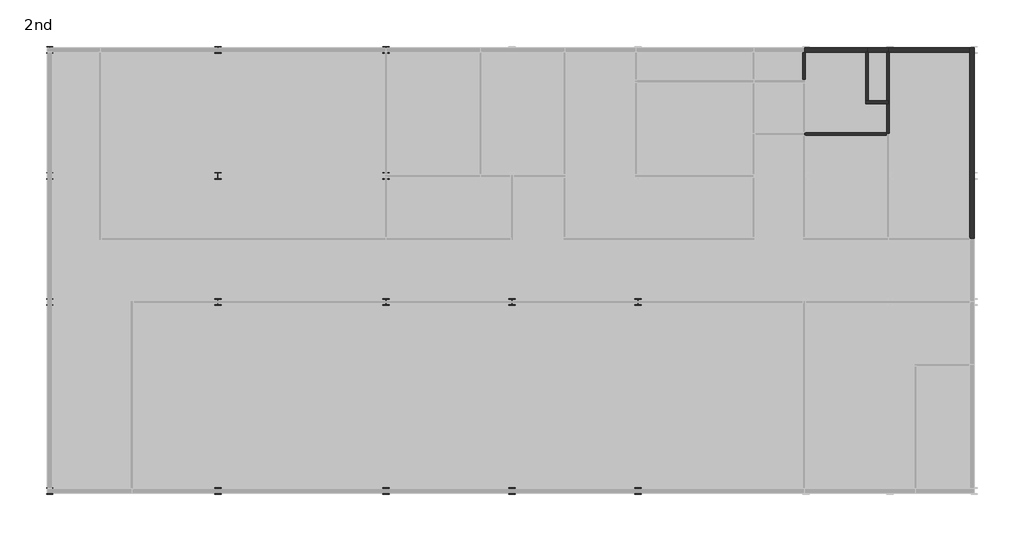
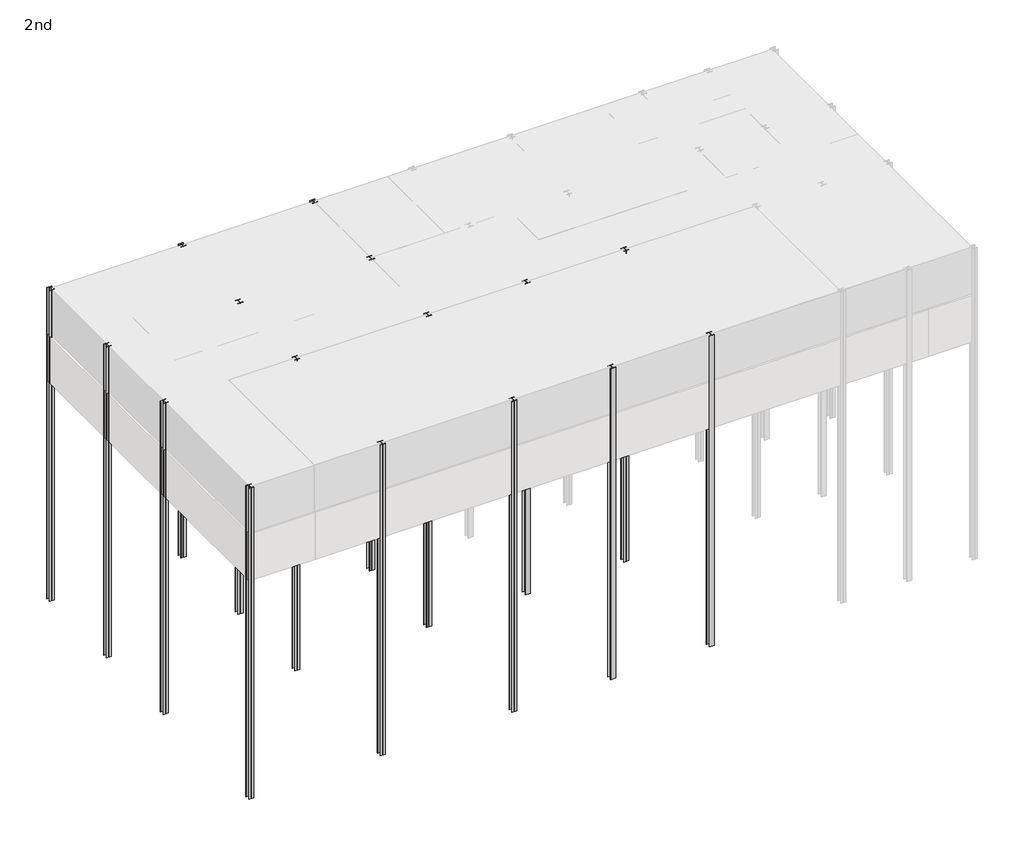
# One storey, part 2 of 3: 16 columns, 10 walls.
"""IFC4 building model written with IfcOpenShell, lengths in millimetres."""

from ifc_helpers import new_model, si_unit, point, frame_2d, origin, origin_with_axes, place, context, project, spatial, polyline, circle_curve, trimmed, segment, composite_curve, outline, extrude, faceted_brep, element, save

model = new_model("IFC4")

# Units and contexts
model_context = context("Model", 3, world=origin())
ifc_project = project(units=[si_unit("LENGTHUNIT", "METRE", prefix="MILLI")], contexts=[model_context])

# Site, building, storey
site = spatial("IfcSite", under=ifc_project)
building = spatial("IfcBuilding", under=site)
storey = spatial("IfcBuildingStorey", under=building, Name="2nd", Elevation=14000.0)

# Columns
placement = place(None, origin())
element("IfcColumn", 1, ObjectType="UC-Universal Columns-Column : UC305x305x97", at=placement, inside=storey, context=model_context, shape_type="SweptSolid", body=[
    extrude(outline(composite_curve([segment(polyline([(156266.7520501, 152169.7081198), (156266.7520501, 152154.3081198), (156134.2520501, 152154.3081198)]), True, "CONTINUOUS"), segment(trimmed(circle_curve(frame_2d((156134.2520501, 152139.1081198)), 15.2), [point((156134.2520501, 152154.3081198))], [point((156119.0520501, 152139.1081198))], True, "CARTESIAN"), True, "CONTINUOUS"), segment(polyline([(156119.0520501, 152139.1081198), (156119.0520501, 151892.4081198)]), True, "CONTINUOUS"), segment(trimmed(circle_curve(frame_2d((156134.2520501, 151892.4081198)), 15.2), [point((156119.0520501, 151892.4081198))], [point((156134.2520501, 151877.2081198))], True, "CARTESIAN"), True, "CONTINUOUS"), segment(polyline([(156134.2520501, 151877.2081198), (156266.7520501, 151877.2081198), (156266.7520501, 151861.8081198), (155961.4520501, 151861.8081198), (155961.4520501, 151877.2081198), (156093.9520501, 151877.2081198)]), True, "CONTINUOUS"), segment(trimmed(circle_curve(frame_2d((156093.9520501, 151892.4081198)), 15.2), [point((156093.9520501, 151877.2081198))], [point((156109.1520501, 151892.4081198))], True, "CARTESIAN"), True, "CONTINUOUS"), segment(polyline([(156109.1520501, 151892.4081198), (156109.1520501, 152139.1081198)]), True, "CONTINUOUS"), segment(trimmed(circle_curve(frame_2d((156093.9520501, 152139.1081198)), 15.2), [point((156109.1520501, 152139.1081198))], [point((156093.9520501, 152154.3081198))], True, "CARTESIAN"), True, "CONTINUOUS"), segment(polyline([(156093.9520501, 152154.3081198), (155961.4520501, 152154.3081198), (155961.4520501, 152169.7081198), (156266.7520501, 152169.7081198)]), True, "CONTINUOUS")], self_intersect=False)), origin_with_axes(), (0.0, 0.0, 1.0), 20000.0),
])
element("IfcColumn", 2, ObjectType="UC-Universal Columns-Column : UC305x305x97", at=placement, inside=storey, context=model_context, shape_type="SweptSolid", body=[
    extrude(outline(composite_curve([segment(polyline([(156266.7520501, 146169.7081198), (156266.7520501, 146154.3081198), (156134.2520501, 146154.3081198)]), True, "CONTINUOUS"), segment(trimmed(circle_curve(frame_2d((156134.2520501, 146139.1081198)), 15.2), [point((156134.2520501, 146154.3081198))], [point((156119.0520501, 146139.1081198))], True, "CARTESIAN"), True, "CONTINUOUS"), segment(polyline([(156119.0520501, 146139.1081198), (156119.0520501, 145892.4081198)]), True, "CONTINUOUS"), segment(trimmed(circle_curve(frame_2d((156134.2520501, 145892.4081198)), 15.2), [point((156119.0520501, 145892.4081198))], [point((156134.2520501, 145877.2081198))], True, "CARTESIAN"), True, "CONTINUOUS"), segment(polyline([(156134.2520501, 145877.2081198), (156266.7520501, 145877.2081198), (156266.7520501, 145861.8081198), (155961.4520501, 145861.8081198), (155961.4520501, 145877.2081198), (156093.9520501, 145877.2081198)]), True, "CONTINUOUS"), segment(trimmed(circle_curve(frame_2d((156093.9520501, 145892.4081198)), 15.2), [point((156093.9520501, 145877.2081198))], [point((156109.1520501, 145892.4081198))], True, "CARTESIAN"), True, "CONTINUOUS"), segment(polyline([(156109.1520501, 145892.4081198), (156109.1520501, 146139.1081198)]), True, "CONTINUOUS"), segment(trimmed(circle_curve(frame_2d((156093.9520501, 146139.1081198)), 15.2), [point((156109.1520501, 146139.1081198))], [point((156093.9520501, 146154.3081198))], True, "CARTESIAN"), True, "CONTINUOUS"), segment(polyline([(156093.9520501, 146154.3081198), (155961.4520501, 146154.3081198), (155961.4520501, 146169.7081198), (156266.7520501, 146169.7081198)]), True, "CONTINUOUS")], self_intersect=False)), origin_with_axes(), (0.0, 0.0, 1.0), 20000.0),
])
element("IfcColumn", 3, ObjectType="UC-Universal Columns-Column : UC305x305x97", at=placement, inside=storey, context=model_context, shape_type="SweptSolid", body=[
    extrude(outline(composite_curve([segment(polyline([(156266.7520501, 140169.7081198), (156266.7520501, 140154.3081198), (156134.2520501, 140154.3081198)]), True, "CONTINUOUS"), segment(trimmed(circle_curve(frame_2d((156134.2520501, 140139.1081198)), 15.2), [point((156134.2520501, 140154.3081198))], [point((156119.0520501, 140139.1081198))], True, "CARTESIAN"), True, "CONTINUOUS"), segment(polyline([(156119.0520501, 140139.1081198), (156119.0520501, 139892.4081198)]), True, "CONTINUOUS"), segment(trimmed(circle_curve(frame_2d((156134.2520501, 139892.4081198)), 15.2), [point((156119.0520501, 139892.4081198))], [point((156134.2520501, 139877.2081198))], True, "CARTESIAN"), True, "CONTINUOUS"), segment(polyline([(156134.2520501, 139877.2081198), (156266.7520501, 139877.2081198), (156266.7520501, 139861.8081198), (155961.4520501, 139861.8081198), (155961.4520501, 139877.2081198), (156093.9520501, 139877.2081198)]), True, "CONTINUOUS"), segment(trimmed(circle_curve(frame_2d((156093.9520501, 139892.4081198)), 15.2), [point((156093.9520501, 139877.2081198))], [point((156109.1520501, 139892.4081198))], True, "CARTESIAN"), True, "CONTINUOUS"), segment(polyline([(156109.1520501, 139892.4081198), (156109.1520501, 140139.1081198)]), True, "CONTINUOUS"), segment(trimmed(circle_curve(frame_2d((156093.9520501, 140139.1081198)), 15.2), [point((156109.1520501, 140139.1081198))], [point((156093.9520501, 140154.3081198))], True, "CARTESIAN"), True, "CONTINUOUS"), segment(polyline([(156093.9520501, 140154.3081198), (155961.4520501, 140154.3081198), (155961.4520501, 140169.7081198), (156266.7520501, 140169.7081198)]), True, "CONTINUOUS")], self_intersect=False)), origin_with_axes(), (0.0, 0.0, 1.0), 20000.0),
])
element("IfcColumn", 4, ObjectType="UC-Universal Columns-Column : UC305x305x97", at=placement, inside=storey, context=model_context, shape_type="SweptSolid", body=[
    extrude(outline(composite_curve([segment(polyline([(156266.7520501, 131169.7081198), (156266.7520501, 131154.3081198), (156134.2520501, 131154.3081198)]), True, "CONTINUOUS"), segment(trimmed(circle_curve(frame_2d((156134.2520501, 131139.1081198)), 15.2), [point((156134.2520501, 131154.3081198))], [point((156119.0520501, 131139.1081198))], True, "CARTESIAN"), True, "CONTINUOUS"), segment(polyline([(156119.0520501, 131139.1081198), (156119.0520501, 130892.4081198)]), True, "CONTINUOUS"), segment(trimmed(circle_curve(frame_2d((156134.2520501, 130892.4081198)), 15.2), [point((156119.0520501, 130892.4081198))], [point((156134.2520501, 130877.2081198))], True, "CARTESIAN"), True, "CONTINUOUS"), segment(polyline([(156134.2520501, 130877.2081198), (156266.7520501, 130877.2081198), (156266.7520501, 130861.8081198), (155961.4520501, 130861.8081198), (155961.4520501, 130877.2081198), (156093.9520501, 130877.2081198)]), True, "CONTINUOUS"), segment(trimmed(circle_curve(frame_2d((156093.9520501, 130892.4081198)), 15.2), [point((156093.9520501, 130877.2081198))], [point((156109.1520501, 130892.4081198))], True, "CARTESIAN"), True, "CONTINUOUS"), segment(polyline([(156109.1520501, 130892.4081198), (156109.1520501, 131139.1081198)]), True, "CONTINUOUS"), segment(trimmed(circle_curve(frame_2d((156093.9520501, 131139.1081198)), 15.2), [point((156109.1520501, 131139.1081198))], [point((156093.9520501, 131154.3081198))], True, "CARTESIAN"), True, "CONTINUOUS"), segment(polyline([(156093.9520501, 131154.3081198), (155961.4520501, 131154.3081198), (155961.4520501, 131169.7081198), (156266.7520501, 131169.7081198)]), True, "CONTINUOUS")], self_intersect=False)), origin_with_axes(), (0.0, 0.0, 1.0), 20000.0),
])
element("IfcColumn", 5, ObjectType="UC-Universal Columns-Column : UC305x305x97", at=placement, inside=storey, context=model_context, shape_type="SweptSolid", body=[
    extrude(outline(composite_curve([segment(polyline([(164266.7520501, 152169.7081198), (164266.7520501, 152154.3081198), (164134.2520501, 152154.3081198)]), True, "CONTINUOUS"), segment(trimmed(circle_curve(frame_2d((164134.2520501, 152139.1081198)), 15.2), [point((164134.2520501, 152154.3081198))], [point((164119.0520501, 152139.1081198))], True, "CARTESIAN"), True, "CONTINUOUS"), segment(polyline([(164119.0520501, 152139.1081198), (164119.0520501, 151892.4081198)]), True, "CONTINUOUS"), segment(trimmed(circle_curve(frame_2d((164134.2520501, 151892.4081198)), 15.2), [point((164119.0520501, 151892.4081198))], [point((164134.2520501, 151877.2081198))], True, "CARTESIAN"), True, "CONTINUOUS"), segment(polyline([(164134.2520501, 151877.2081198), (164266.7520501, 151877.2081198), (164266.7520501, 151861.8081198), (163961.4520501, 151861.8081198), (163961.4520501, 151877.2081198), (164093.9520501, 151877.2081198)]), True, "CONTINUOUS"), segment(trimmed(circle_curve(frame_2d((164093.9520501, 151892.4081198)), 15.2), [point((164093.9520501, 151877.2081198))], [point((164109.1520501, 151892.4081198))], True, "CARTESIAN"), True, "CONTINUOUS"), segment(polyline([(164109.1520501, 151892.4081198), (164109.1520501, 152139.1081198)]), True, "CONTINUOUS"), segment(trimmed(circle_curve(frame_2d((164093.9520501, 152139.1081198)), 15.2), [point((164109.1520501, 152139.1081198))], [point((164093.9520501, 152154.3081198))], True, "CARTESIAN"), True, "CONTINUOUS"), segment(polyline([(164093.9520501, 152154.3081198), (163961.4520501, 152154.3081198), (163961.4520501, 152169.7081198), (164266.7520501, 152169.7081198)]), True, "CONTINUOUS")], self_intersect=False)), origin_with_axes(), (0.0, 0.0, 1.0), 20000.0),
])
element("IfcColumn", 6, ObjectType="UC-Universal Columns-Column : UC305x305x97", at=placement, inside=storey, context=model_context, shape_type="SweptSolid", body=[
    extrude(outline(composite_curve([segment(polyline([(164266.7520501, 146169.7081198), (164266.7520501, 146154.3081198), (164134.2520501, 146154.3081198)]), True, "CONTINUOUS"), segment(trimmed(circle_curve(frame_2d((164134.2520501, 146139.1081198)), 15.2), [point((164134.2520501, 146154.3081198))], [point((164119.0520501, 146139.1081198))], True, "CARTESIAN"), True, "CONTINUOUS"), segment(polyline([(164119.0520501, 146139.1081198), (164119.0520501, 145892.4081198)]), True, "CONTINUOUS"), segment(trimmed(circle_curve(frame_2d((164134.2520501, 145892.4081198)), 15.2), [point((164119.0520501, 145892.4081198))], [point((164134.2520501, 145877.2081198))], True, "CARTESIAN"), True, "CONTINUOUS"), segment(polyline([(164134.2520501, 145877.2081198), (164266.7520501, 145877.2081198), (164266.7520501, 145861.8081198), (163961.4520501, 145861.8081198), (163961.4520501, 145877.2081198), (164093.9520501, 145877.2081198)]), True, "CONTINUOUS"), segment(trimmed(circle_curve(frame_2d((164093.9520501, 145892.4081198)), 15.2), [point((164093.9520501, 145877.2081198))], [point((164109.1520501, 145892.4081198))], True, "CARTESIAN"), True, "CONTINUOUS"), segment(polyline([(164109.1520501, 145892.4081198), (164109.1520501, 146139.1081198)]), True, "CONTINUOUS"), segment(trimmed(circle_curve(frame_2d((164093.9520501, 146139.1081198)), 15.2), [point((164109.1520501, 146139.1081198))], [point((164093.9520501, 146154.3081198))], True, "CARTESIAN"), True, "CONTINUOUS"), segment(polyline([(164093.9520501, 146154.3081198), (163961.4520501, 146154.3081198), (163961.4520501, 146169.7081198), (164266.7520501, 146169.7081198)]), True, "CONTINUOUS")], self_intersect=False)), origin_with_axes(), (0.0, 0.0, 1.0), 20000.0),
])
element("IfcColumn", 7, ObjectType="UC-Universal Columns-Column : UC305x305x97", at=placement, inside=storey, context=model_context, shape_type="SweptSolid", body=[
    extrude(outline(composite_curve([segment(polyline([(164266.7520501, 140169.7081198), (164266.7520501, 140154.3081198), (164134.2520501, 140154.3081198)]), True, "CONTINUOUS"), segment(trimmed(circle_curve(frame_2d((164134.2520501, 140139.1081198)), 15.2), [point((164134.2520501, 140154.3081198))], [point((164119.0520501, 140139.1081198))], True, "CARTESIAN"), True, "CONTINUOUS"), segment(polyline([(164119.0520501, 140139.1081198), (164119.0520501, 139892.4081198)]), True, "CONTINUOUS"), segment(trimmed(circle_curve(frame_2d((164134.2520501, 139892.4081198)), 15.2), [point((164119.0520501, 139892.4081198))], [point((164134.2520501, 139877.2081198))], True, "CARTESIAN"), True, "CONTINUOUS"), segment(polyline([(164134.2520501, 139877.2081198), (164266.7520501, 139877.2081198), (164266.7520501, 139861.8081198), (163961.4520501, 139861.8081198), (163961.4520501, 139877.2081198), (164093.9520501, 139877.2081198)]), True, "CONTINUOUS"), segment(trimmed(circle_curve(frame_2d((164093.9520501, 139892.4081198)), 15.2), [point((164093.9520501, 139877.2081198))], [point((164109.1520501, 139892.4081198))], True, "CARTESIAN"), True, "CONTINUOUS"), segment(polyline([(164109.1520501, 139892.4081198), (164109.1520501, 140139.1081198)]), True, "CONTINUOUS"), segment(trimmed(circle_curve(frame_2d((164093.9520501, 140139.1081198)), 15.2), [point((164109.1520501, 140139.1081198))], [point((164093.9520501, 140154.3081198))], True, "CARTESIAN"), True, "CONTINUOUS"), segment(polyline([(164093.9520501, 140154.3081198), (163961.4520501, 140154.3081198), (163961.4520501, 140169.7081198), (164266.7520501, 140169.7081198)]), True, "CONTINUOUS")], self_intersect=False)), origin_with_axes(), (0.0, 0.0, 1.0), 20000.0),
])
element("IfcColumn", 8, ObjectType="UC-Universal Columns-Column : UC305x305x97", at=placement, inside=storey, context=model_context, shape_type="SweptSolid", body=[
    extrude(outline(composite_curve([segment(polyline([(164266.7520501, 131169.7081198), (164266.7520501, 131154.3081198), (164134.2520501, 131154.3081198)]), True, "CONTINUOUS"), segment(trimmed(circle_curve(frame_2d((164134.2520501, 131139.1081198)), 15.2), [point((164134.2520501, 131154.3081198))], [point((164119.0520501, 131139.1081198))], True, "CARTESIAN"), True, "CONTINUOUS"), segment(polyline([(164119.0520501, 131139.1081198), (164119.0520501, 130892.4081198)]), True, "CONTINUOUS"), segment(trimmed(circle_curve(frame_2d((164134.2520501, 130892.4081198)), 15.2), [point((164119.0520501, 130892.4081198))], [point((164134.2520501, 130877.2081198))], True, "CARTESIAN"), True, "CONTINUOUS"), segment(polyline([(164134.2520501, 130877.2081198), (164266.7520501, 130877.2081198), (164266.7520501, 130861.8081198), (163961.4520501, 130861.8081198), (163961.4520501, 130877.2081198), (164093.9520501, 130877.2081198)]), True, "CONTINUOUS"), segment(trimmed(circle_curve(frame_2d((164093.9520501, 130892.4081198)), 15.2), [point((164093.9520501, 130877.2081198))], [point((164109.1520501, 130892.4081198))], True, "CARTESIAN"), True, "CONTINUOUS"), segment(polyline([(164109.1520501, 130892.4081198), (164109.1520501, 131139.1081198)]), True, "CONTINUOUS"), segment(trimmed(circle_curve(frame_2d((164093.9520501, 131139.1081198)), 15.2), [point((164109.1520501, 131139.1081198))], [point((164093.9520501, 131154.3081198))], True, "CARTESIAN"), True, "CONTINUOUS"), segment(polyline([(164093.9520501, 131154.3081198), (163961.4520501, 131154.3081198), (163961.4520501, 131169.7081198), (164266.7520501, 131169.7081198)]), True, "CONTINUOUS")], self_intersect=False)), origin_with_axes(), (0.0, 0.0, 1.0), 20000.0),
])
element("IfcColumn", 9, ObjectType="UC-Universal Columns-Column : UC305x305x97", at=placement, inside=storey, context=model_context, shape_type="SweptSolid", body=[
    extrude(outline(composite_curve([segment(polyline([(172266.7520501, 152169.7081198), (172266.7520501, 152154.3081198), (172134.2520501, 152154.3081198)]), True, "CONTINUOUS"), segment(trimmed(circle_curve(frame_2d((172134.2520501, 152139.1081198)), 15.2), [point((172134.2520501, 152154.3081198))], [point((172119.0520501, 152139.1081198))], True, "CARTESIAN"), True, "CONTINUOUS"), segment(polyline([(172119.0520501, 152139.1081198), (172119.0520501, 151892.4081198)]), True, "CONTINUOUS"), segment(trimmed(circle_curve(frame_2d((172134.2520501, 151892.4081198)), 15.2), [point((172119.0520501, 151892.4081198))], [point((172134.2520501, 151877.2081198))], True, "CARTESIAN"), True, "CONTINUOUS"), segment(polyline([(172134.2520501, 151877.2081198), (172266.7520501, 151877.2081198), (172266.7520501, 151861.8081198), (171961.4520501, 151861.8081198), (171961.4520501, 151877.2081198), (172093.9520501, 151877.2081198)]), True, "CONTINUOUS"), segment(trimmed(circle_curve(frame_2d((172093.9520501, 151892.4081198)), 15.2), [point((172093.9520501, 151877.2081198))], [point((172109.1520501, 151892.4081198))], True, "CARTESIAN"), True, "CONTINUOUS"), segment(polyline([(172109.1520501, 151892.4081198), (172109.1520501, 152139.1081198)]), True, "CONTINUOUS"), segment(trimmed(circle_curve(frame_2d((172093.9520501, 152139.1081198)), 15.2), [point((172109.1520501, 152139.1081198))], [point((172093.9520501, 152154.3081198))], True, "CARTESIAN"), True, "CONTINUOUS"), segment(polyline([(172093.9520501, 152154.3081198), (171961.4520501, 152154.3081198), (171961.4520501, 152169.7081198), (172266.7520501, 152169.7081198)]), True, "CONTINUOUS")], self_intersect=False)), origin_with_axes(), (0.0, 0.0, 1.0), 20000.0),
])
element("IfcColumn", 10, ObjectType="UC-Universal Columns-Column : UC305x305x97", at=placement, inside=storey, context=model_context, shape_type="SweptSolid", body=[
    extrude(outline(composite_curve([segment(polyline([(172266.7520501, 146169.7081198), (172266.7520501, 146154.3081198), (172134.2520501, 146154.3081198)]), True, "CONTINUOUS"), segment(trimmed(circle_curve(frame_2d((172134.2520501, 146139.1081198)), 15.2), [point((172134.2520501, 146154.3081198))], [point((172119.0520501, 146139.1081198))], True, "CARTESIAN"), True, "CONTINUOUS"), segment(polyline([(172119.0520501, 146139.1081198), (172119.0520501, 145892.4081198)]), True, "CONTINUOUS"), segment(trimmed(circle_curve(frame_2d((172134.2520501, 145892.4081198)), 15.2), [point((172119.0520501, 145892.4081198))], [point((172134.2520501, 145877.2081198))], True, "CARTESIAN"), True, "CONTINUOUS"), segment(polyline([(172134.2520501, 145877.2081198), (172266.7520501, 145877.2081198), (172266.7520501, 145861.8081198), (171961.4520501, 145861.8081198), (171961.4520501, 145877.2081198), (172093.9520501, 145877.2081198)]), True, "CONTINUOUS"), segment(trimmed(circle_curve(frame_2d((172093.9520501, 145892.4081198)), 15.2), [point((172093.9520501, 145877.2081198))], [point((172109.1520501, 145892.4081198))], True, "CARTESIAN"), True, "CONTINUOUS"), segment(polyline([(172109.1520501, 145892.4081198), (172109.1520501, 146139.1081198)]), True, "CONTINUOUS"), segment(trimmed(circle_curve(frame_2d((172093.9520501, 146139.1081198)), 15.2), [point((172109.1520501, 146139.1081198))], [point((172093.9520501, 146154.3081198))], True, "CARTESIAN"), True, "CONTINUOUS"), segment(polyline([(172093.9520501, 146154.3081198), (171961.4520501, 146154.3081198), (171961.4520501, 146169.7081198), (172266.7520501, 146169.7081198)]), True, "CONTINUOUS")], self_intersect=False)), origin_with_axes(), (0.0, 0.0, 1.0), 20000.0),
])
element("IfcColumn", 11, ObjectType="UC-Universal Columns-Column : UC305x305x97", at=placement, inside=storey, context=model_context, shape_type="SweptSolid", body=[
    extrude(outline(composite_curve([segment(polyline([(172266.7520501, 140169.7081198), (172266.7520501, 140154.3081198), (172134.2520501, 140154.3081198)]), True, "CONTINUOUS"), segment(trimmed(circle_curve(frame_2d((172134.2520501, 140139.1081198)), 15.2), [point((172134.2520501, 140154.3081198))], [point((172119.0520501, 140139.1081198))], True, "CARTESIAN"), True, "CONTINUOUS"), segment(polyline([(172119.0520501, 140139.1081198), (172119.0520501, 139892.4081198)]), True, "CONTINUOUS"), segment(trimmed(circle_curve(frame_2d((172134.2520501, 139892.4081198)), 15.2), [point((172119.0520501, 139892.4081198))], [point((172134.2520501, 139877.2081198))], True, "CARTESIAN"), True, "CONTINUOUS"), segment(polyline([(172134.2520501, 139877.2081198), (172266.7520501, 139877.2081198), (172266.7520501, 139861.8081198), (171961.4520501, 139861.8081198), (171961.4520501, 139877.2081198), (172093.9520501, 139877.2081198)]), True, "CONTINUOUS"), segment(trimmed(circle_curve(frame_2d((172093.9520501, 139892.4081198)), 15.2), [point((172093.9520501, 139877.2081198))], [point((172109.1520501, 139892.4081198))], True, "CARTESIAN"), True, "CONTINUOUS"), segment(polyline([(172109.1520501, 139892.4081198), (172109.1520501, 140139.1081198)]), True, "CONTINUOUS"), segment(trimmed(circle_curve(frame_2d((172093.9520501, 140139.1081198)), 15.2), [point((172109.1520501, 140139.1081198))], [point((172093.9520501, 140154.3081198))], True, "CARTESIAN"), True, "CONTINUOUS"), segment(polyline([(172093.9520501, 140154.3081198), (171961.4520501, 140154.3081198), (171961.4520501, 140169.7081198), (172266.7520501, 140169.7081198)]), True, "CONTINUOUS")], self_intersect=False)), origin_with_axes(), (0.0, 0.0, 1.0), 20000.0),
])
element("IfcColumn", 12, ObjectType="UC-Universal Columns-Column : UC305x305x97", at=placement, inside=storey, context=model_context, shape_type="SweptSolid", body=[
    extrude(outline(composite_curve([segment(polyline([(172266.7520501, 131169.7081198), (172266.7520501, 131154.3081198), (172134.2520501, 131154.3081198)]), True, "CONTINUOUS"), segment(trimmed(circle_curve(frame_2d((172134.2520501, 131139.1081198)), 15.2), [point((172134.2520501, 131154.3081198))], [point((172119.0520501, 131139.1081198))], True, "CARTESIAN"), True, "CONTINUOUS"), segment(polyline([(172119.0520501, 131139.1081198), (172119.0520501, 130892.4081198)]), True, "CONTINUOUS"), segment(trimmed(circle_curve(frame_2d((172134.2520501, 130892.4081198)), 15.2), [point((172119.0520501, 130892.4081198))], [point((172134.2520501, 130877.2081198))], True, "CARTESIAN"), True, "CONTINUOUS"), segment(polyline([(172134.2520501, 130877.2081198), (172266.7520501, 130877.2081198), (172266.7520501, 130861.8081198), (171961.4520501, 130861.8081198), (171961.4520501, 130877.2081198), (172093.9520501, 130877.2081198)]), True, "CONTINUOUS"), segment(trimmed(circle_curve(frame_2d((172093.9520501, 130892.4081198)), 15.2), [point((172093.9520501, 130877.2081198))], [point((172109.1520501, 130892.4081198))], True, "CARTESIAN"), True, "CONTINUOUS"), segment(polyline([(172109.1520501, 130892.4081198), (172109.1520501, 131139.1081198)]), True, "CONTINUOUS"), segment(trimmed(circle_curve(frame_2d((172093.9520501, 131139.1081198)), 15.2), [point((172109.1520501, 131139.1081198))], [point((172093.9520501, 131154.3081198))], True, "CARTESIAN"), True, "CONTINUOUS"), segment(polyline([(172093.9520501, 131154.3081198), (171961.4520501, 131154.3081198), (171961.4520501, 131169.7081198), (172266.7520501, 131169.7081198)]), True, "CONTINUOUS")], self_intersect=False)), origin_with_axes(), (0.0, 0.0, 1.0), 20000.0),
])
element("IfcColumn", 13, ObjectType="UC-Universal Columns-Column : UC305x305x97", at=placement, inside=storey, context=model_context, shape_type="SweptSolid", body=[
    extrude(outline(composite_curve([segment(polyline([(178266.7520501, 140169.7081198), (178266.7520501, 140154.3081198), (178134.2520501, 140154.3081198)]), True, "CONTINUOUS"), segment(trimmed(circle_curve(frame_2d((178134.2520501, 140139.1081198)), 15.2), [point((178134.2520501, 140154.3081198))], [point((178119.0520501, 140139.1081198))], True, "CARTESIAN"), True, "CONTINUOUS"), segment(polyline([(178119.0520501, 140139.1081198), (178119.0520501, 139892.4081198)]), True, "CONTINUOUS"), segment(trimmed(circle_curve(frame_2d((178134.2520501, 139892.4081198)), 15.2), [point((178119.0520501, 139892.4081198))], [point((178134.2520501, 139877.2081198))], True, "CARTESIAN"), True, "CONTINUOUS"), segment(polyline([(178134.2520501, 139877.2081198), (178266.7520501, 139877.2081198), (178266.7520501, 139861.8081198), (177961.4520501, 139861.8081198), (177961.4520501, 139877.2081198), (178093.9520501, 139877.2081198)]), True, "CONTINUOUS"), segment(trimmed(circle_curve(frame_2d((178093.9520501, 139892.4081198)), 15.2), [point((178093.9520501, 139877.2081198))], [point((178109.1520501, 139892.4081198))], True, "CARTESIAN"), True, "CONTINUOUS"), segment(polyline([(178109.1520501, 139892.4081198), (178109.1520501, 140139.1081198)]), True, "CONTINUOUS"), segment(trimmed(circle_curve(frame_2d((178093.9520501, 140139.1081198)), 15.2), [point((178109.1520501, 140139.1081198))], [point((178093.9520501, 140154.3081198))], True, "CARTESIAN"), True, "CONTINUOUS"), segment(polyline([(178093.9520501, 140154.3081198), (177961.4520501, 140154.3081198), (177961.4520501, 140169.7081198), (178266.7520501, 140169.7081198)]), True, "CONTINUOUS")], self_intersect=False)), origin_with_axes(), (0.0, 0.0, 1.0), 20000.0),
])
element("IfcColumn", 14, ObjectType="UC-Universal Columns-Column : UC305x305x97", at=placement, inside=storey, context=model_context, shape_type="SweptSolid", body=[
    extrude(outline(composite_curve([segment(polyline([(178266.7520501, 131169.7081198), (178266.7520501, 131154.3081198), (178134.2520501, 131154.3081198)]), True, "CONTINUOUS"), segment(trimmed(circle_curve(frame_2d((178134.2520501, 131139.1081198)), 15.2), [point((178134.2520501, 131154.3081198))], [point((178119.0520501, 131139.1081198))], True, "CARTESIAN"), True, "CONTINUOUS"), segment(polyline([(178119.0520501, 131139.1081198), (178119.0520501, 130892.4081198)]), True, "CONTINUOUS"), segment(trimmed(circle_curve(frame_2d((178134.2520501, 130892.4081198)), 15.2), [point((178119.0520501, 130892.4081198))], [point((178134.2520501, 130877.2081198))], True, "CARTESIAN"), True, "CONTINUOUS"), segment(polyline([(178134.2520501, 130877.2081198), (178266.7520501, 130877.2081198), (178266.7520501, 130861.8081198), (177961.4520501, 130861.8081198), (177961.4520501, 130877.2081198), (178093.9520501, 130877.2081198)]), True, "CONTINUOUS"), segment(trimmed(circle_curve(frame_2d((178093.9520501, 130892.4081198)), 15.2), [point((178093.9520501, 130877.2081198))], [point((178109.1520501, 130892.4081198))], True, "CARTESIAN"), True, "CONTINUOUS"), segment(polyline([(178109.1520501, 130892.4081198), (178109.1520501, 131139.1081198)]), True, "CONTINUOUS"), segment(trimmed(circle_curve(frame_2d((178093.9520501, 131139.1081198)), 15.2), [point((178109.1520501, 131139.1081198))], [point((178093.9520501, 131154.3081198))], True, "CARTESIAN"), True, "CONTINUOUS"), segment(polyline([(178093.9520501, 131154.3081198), (177961.4520501, 131154.3081198), (177961.4520501, 131169.7081198), (178266.7520501, 131169.7081198)]), True, "CONTINUOUS")], self_intersect=False)), origin_with_axes(), (0.0, 0.0, 1.0), 20000.0),
])
element("IfcColumn", 15, ObjectType="UC-Universal Columns-Column : UC305x305x97", at=placement, inside=storey, context=model_context, shape_type="SweptSolid", body=[
    extrude(outline(composite_curve([segment(polyline([(184266.7520501, 140169.7081198), (184266.7520501, 140154.3081198), (184134.2520501, 140154.3081198)]), True, "CONTINUOUS"), segment(trimmed(circle_curve(frame_2d((184134.2520501, 140139.1081198)), 15.2), [point((184134.2520501, 140154.3081198))], [point((184119.0520501, 140139.1081198))], True, "CARTESIAN"), True, "CONTINUOUS"), segment(polyline([(184119.0520501, 140139.1081198), (184119.0520501, 139892.4081198)]), True, "CONTINUOUS"), segment(trimmed(circle_curve(frame_2d((184134.2520501, 139892.4081198)), 15.2), [point((184119.0520501, 139892.4081198))], [point((184134.2520501, 139877.2081198))], True, "CARTESIAN"), True, "CONTINUOUS"), segment(polyline([(184134.2520501, 139877.2081198), (184266.7520501, 139877.2081198), (184266.7520501, 139861.8081198), (183961.4520501, 139861.8081198), (183961.4520501, 139877.2081198), (184093.9520501, 139877.2081198)]), True, "CONTINUOUS"), segment(trimmed(circle_curve(frame_2d((184093.9520501, 139892.4081198)), 15.2), [point((184093.9520501, 139877.2081198))], [point((184109.1520501, 139892.4081198))], True, "CARTESIAN"), True, "CONTINUOUS"), segment(polyline([(184109.1520501, 139892.4081198), (184109.1520501, 140139.1081198)]), True, "CONTINUOUS"), segment(trimmed(circle_curve(frame_2d((184093.9520501, 140139.1081198)), 15.2), [point((184109.1520501, 140139.1081198))], [point((184093.9520501, 140154.3081198))], True, "CARTESIAN"), True, "CONTINUOUS"), segment(polyline([(184093.9520501, 140154.3081198), (183961.4520501, 140154.3081198), (183961.4520501, 140169.7081198), (184266.7520501, 140169.7081198)]), True, "CONTINUOUS")], self_intersect=False)), origin_with_axes(), (0.0, 0.0, 1.0), 20000.0),
])
element("IfcColumn", 16, ObjectType="UC-Universal Columns-Column : UC305x305x97", at=placement, inside=storey, context=model_context, shape_type="SweptSolid", body=[
    extrude(outline(composite_curve([segment(polyline([(184266.7520501, 131169.7081198), (184266.7520501, 131154.3081198), (184134.2520501, 131154.3081198)]), True, "CONTINUOUS"), segment(trimmed(circle_curve(frame_2d((184134.2520501, 131139.1081198)), 15.2), [point((184134.2520501, 131154.3081198))], [point((184119.0520501, 131139.1081198))], True, "CARTESIAN"), True, "CONTINUOUS"), segment(polyline([(184119.0520501, 131139.1081198), (184119.0520501, 130892.4081198)]), True, "CONTINUOUS"), segment(trimmed(circle_curve(frame_2d((184134.2520501, 130892.4081198)), 15.2), [point((184119.0520501, 130892.4081198))], [point((184134.2520501, 130877.2081198))], True, "CARTESIAN"), True, "CONTINUOUS"), segment(polyline([(184134.2520501, 130877.2081198), (184266.7520501, 130877.2081198), (184266.7520501, 130861.8081198), (183961.4520501, 130861.8081198), (183961.4520501, 130877.2081198), (184093.9520501, 130877.2081198)]), True, "CONTINUOUS"), segment(trimmed(circle_curve(frame_2d((184093.9520501, 130892.4081198)), 15.2), [point((184093.9520501, 130877.2081198))], [point((184109.1520501, 130892.4081198))], True, "CARTESIAN"), True, "CONTINUOUS"), segment(polyline([(184109.1520501, 130892.4081198), (184109.1520501, 131139.1081198)]), True, "CONTINUOUS"), segment(trimmed(circle_curve(frame_2d((184093.9520501, 131139.1081198)), 15.2), [point((184109.1520501, 131139.1081198))], [point((184093.9520501, 131154.3081198))], True, "CARTESIAN"), True, "CONTINUOUS"), segment(polyline([(184093.9520501, 131154.3081198), (183961.4520501, 131154.3081198), (183961.4520501, 131169.7081198), (184266.7520501, 131169.7081198)]), True, "CONTINUOUS")], self_intersect=False)), origin_with_axes(), (0.0, 0.0, 1.0), 20000.0),
])

# Walls
element("IfcWall", 17, ObjectType="Wall-Ext_215Bwk", at=placement, inside=storey, context=model_context, shape_type="Brep", body=[
    faceted_brep([(200121.6020501, 143015.7581198, 14000.0), (200121.6020501, 152123.2581198, 14000.0), (200121.6020501, 152123.2581198, 17000.0), (200121.6020501, 143015.7581198, 17000.0), (199906.6020501, 143015.7581198, 14000.0), (199906.6020501, 143015.7581198, 17000.0), (199906.6020501, 143078.2581198, 17000.0), (199906.6020501, 151908.2581198, 17000.0), (199906.6020501, 152123.2581198, 17000.0), (199906.6020501, 152123.2581198, 14000.0), (199906.6020501, 151908.2581198, 14000.0), (199906.6020501, 143078.2581198, 14000.0)], [[[0, 1, 2, 3]], [[4, 5, 6, 7, 8, 9, 10, 11]], [[1, 0, 4, 11, 10, 9]], [[3, 2, 8, 7, 6, 5]], [[0, 3, 5, 4]], [[2, 1, 9, 8]]]),
])
element("IfcWall", 18, ObjectType="Wall-Ext_215Bwk", at=placement, inside=storey, context=model_context, shape_type="Brep", body=[
    faceted_brep([(199906.6020501, 152123.2581198, 14000.0), (196014.1020501, 152123.2581198, 14000.0), (196014.1020501, 152123.2581198, 17000.0), (199906.6020501, 152123.2581198, 17000.0), (199906.6020501, 151908.2581198, 14000.0), (199906.6020501, 151908.2581198, 17000.0), (196076.6020501, 151908.2581198, 17000.0), (196014.1020501, 151908.2581198, 17000.0), (196014.1020501, 151908.2581198, 14000.0), (196076.6020501, 151908.2581198, 14000.0)], [[[0, 1, 2, 3]], [[4, 5, 6, 7, 8, 9]], [[1, 0, 4, 9, 8]], [[2, 1, 8, 7]], [[3, 2, 7, 6, 5]], [[0, 3, 5, 4]]]),
])
element("IfcWall", 19, ObjectType="Wall-Ext_215Bwk", at=placement, inside=storey, context=model_context, shape_type="Brep", body=[
    faceted_brep([(195014.1020501, 152123.2581198, 14000.0), (192014.1020501, 152123.2581198, 14000.0), (192014.1020501, 152123.2581198, 17000.0), (195014.1020501, 152123.2581198, 17000.0), (195014.1020501, 151908.2581198, 14000.0), (195014.1020501, 151908.2581198, 17000.0), (194951.6020501, 151908.2581198, 17000.0), (192076.6020501, 151908.2581198, 17000.0), (192014.1020501, 151908.2581198, 17000.0), (192014.1020501, 151908.2581198, 14000.0), (192076.6020501, 151908.2581198, 14000.0), (194951.6020501, 151908.2581198, 14000.0)], [[[0, 1, 2, 3]], [[4, 5, 6, 7, 8, 9, 10, 11]], [[1, 0, 4, 11, 10, 9]], [[2, 1, 9, 8]], [[3, 2, 8, 7, 6, 5]], [[0, 3, 5, 4]]]),
])
element("IfcWall", 20, ObjectType="Wall-Ext_215Bwk", at=placement, inside=storey, context=model_context, shape_type="Brep", body=[
    faceted_brep([(196014.1020501, 152123.2581198, 14000.0), (195014.1020501, 152123.2581198, 14000.0), (195014.1020501, 152123.2581198, 17000.0), (196014.1020501, 152123.2581198, 17000.0), (196014.1020501, 151908.2581198, 14000.0), (196014.1020501, 151908.2581198, 17000.0), (195951.6020501, 151908.2581198, 17000.0), (195076.6020501, 151908.2581198, 17000.0), (195014.1020501, 151908.2581198, 17000.0), (195014.1020501, 151908.2581198, 14000.0), (195076.6020501, 151908.2581198, 14000.0), (195951.6020501, 151908.2581198, 14000.0)], [[[0, 1, 2, 3]], [[4, 5, 6, 7, 8, 9, 10, 11]], [[1, 0, 4, 11, 10, 9]], [[2, 1, 9, 8]], [[3, 2, 8, 7, 6, 5]], [[0, 3, 5, 4]]]),
])
element("IfcWall", 21, ObjectType="Wall-Int_12P-100Blk-12P", at=placement, inside=storey, context=model_context, shape_type="Brep", body=[
    faceted_brep([(195951.6020501, 148078.2581198, 14000.0), (192076.6020501, 148078.2581198, 14000.0), (192014.1020501, 148078.2581198, 14000.0), (192014.1020501, 148078.2581198, 17000.0), (192076.6020501, 148078.2581198, 17000.0), (195951.6020501, 148078.2581198, 17000.0), (195951.6020501, 147953.2581198, 14000.0), (195951.6020501, 147953.2581198, 17000.0), (192076.6020501, 147953.2581198, 17000.0), (192014.1020501, 147953.2581198, 17000.0), (192014.1020501, 147953.2581198, 14000.0), (192076.6020501, 147953.2581198, 14000.0), (195951.6020501, 148015.7581198, 14000.0), (195951.6020501, 148015.7581198, 17000.0)], [[[0, 1, 2, 3, 4, 5]], [[6, 7, 8, 9, 10, 11]], [[2, 1, 0, 12, 6, 11, 10]], [[3, 2, 10, 9]], [[5, 4, 3, 9, 8, 7, 13]], [[0, 5, 13, 7, 6, 12]]]),
])
element("IfcWall", 22, ObjectType="Wall-Int_12P-100Blk-12P", at=placement, inside=storey, context=model_context, shape_type="Brep", body=[
    faceted_brep([(195951.6020501, 151908.2581198, 14000.0), (195951.6020501, 149515.7581198, 14000.0), (195951.6020501, 149515.7581198, 17000.0), (195951.6020501, 151908.2581198, 17000.0), (196076.6020501, 151908.2581198, 14000.0), (196076.6020501, 151908.2581198, 17000.0), (196076.6020501, 149515.7581198, 17000.0), (196076.6020501, 149515.7581198, 14000.0), (196014.1020501, 151908.2581198, 14000.0), (196014.1020501, 151908.2581198, 17000.0)], [[[0, 1, 2, 3]], [[4, 5, 6, 7]], [[1, 0, 8, 4, 7]], [[2, 1, 7, 6]], [[3, 2, 6, 5, 9]], [[0, 3, 9, 5, 4, 8]]]),
])
element("IfcWall", 23, ObjectType="Wall-Int_12P-100Blk-12P", at=placement, inside=storey, context=model_context, shape_type="Brep", body=[
    faceted_brep([(195951.6020501, 149515.7581198, 14000.0), (195951.6020501, 148078.2581198, 14000.0), (195951.6020501, 148015.7581198, 14000.0), (195951.6020501, 148015.7581198, 17000.0), (195951.6020501, 148078.2581198, 17000.0), (195951.6020501, 149515.7581198, 17000.0), (196076.6020501, 149515.7581198, 14000.0), (196076.6020501, 149515.7581198, 17000.0), (196076.6020501, 148015.7581198, 17000.0), (196076.6020501, 148015.7581198, 14000.0)], [[[0, 1, 2, 3, 4, 5]], [[6, 7, 8, 9]], [[2, 1, 0, 6, 9]], [[3, 2, 9, 8]], [[5, 4, 3, 8, 7]], [[0, 5, 7, 6]]]),
])
element("IfcWall", 24, ObjectType="Wall-Int_12P-100Blk-12P", at=placement, inside=storey, context=model_context, shape_type="Brep", body=[
    faceted_brep([(192076.6020501, 150578.2581198, 14000.0), (192076.6020501, 151908.2581198, 14000.0), (192076.6020501, 151908.2581198, 17000.0), (192076.6020501, 150578.2581198, 17000.0), (191951.6020501, 150578.2581198, 14000.0), (191951.6020501, 150578.2581198, 17000.0), (191951.6020501, 151908.2581198, 17000.0), (191951.6020501, 151908.2581198, 14000.0), (192014.1020501, 151908.2581198, 14000.0), (192014.1020501, 151908.2581198, 17000.0)], [[[0, 1, 2, 3]], [[4, 5, 6, 7]], [[1, 0, 4, 7, 8]], [[3, 2, 9, 6, 5]], [[2, 1, 8, 7, 6, 9]], [[0, 3, 5, 4]]]),
])
element("IfcWall", 25, ObjectType="Wall-Int_12P-100Blk-12P", at=placement, inside=storey, context=model_context, shape_type="Brep", body=[
    faceted_brep([(196014.1020501, 149578.2581198, 14000.0), (195076.6020501, 149578.2581198, 14000.0), (194951.6020501, 149578.2581198, 14000.0), (194951.6020501, 149578.2581198, 17000.0), (195076.6020501, 149578.2581198, 17000.0), (196014.1020501, 149578.2581198, 17000.0), (196014.1020501, 149453.2581198, 14000.0), (196014.1020501, 149453.2581198, 17000.0), (194951.6020501, 149453.2581198, 17000.0), (194951.6020501, 149453.2581198, 14000.0)], [[[0, 1, 2, 3, 4, 5]], [[6, 7, 8, 9]], [[2, 1, 0, 6, 9]], [[5, 4, 3, 8, 7]], [[0, 5, 7, 6]], [[3, 2, 9, 8]]]),
])
element("IfcWall", 26, ObjectType="Wall-Int_12P-100Blk-12P", at=placement, inside=storey, context=model_context, shape_type="Brep", body=[
    faceted_brep([(195076.6020501, 149578.2581198, 14000.0), (195076.6020501, 151908.2581198, 14000.0), (195076.6020501, 151908.2581198, 17000.0), (195076.6020501, 149578.2581198, 17000.0), (194951.6020501, 149578.2581198, 14000.0), (194951.6020501, 149578.2581198, 17000.0), (194951.6020501, 151908.2581198, 17000.0), (194951.6020501, 151908.2581198, 14000.0), (195014.1020501, 151908.2581198, 14000.0), (195014.1020501, 151908.2581198, 17000.0)], [[[0, 1, 2, 3]], [[4, 5, 6, 7]], [[1, 0, 4, 7, 8]], [[3, 2, 9, 6, 5]], [[2, 1, 8, 7, 6, 9]], [[0, 3, 5, 4]]]),
])

save(model, "model.ifc")

# Revit data of these elements
# Type "UC-Universal Columns-Column : UC305x305x97"
#   Section Name Key = "UC305x305x97"
#   Width = 30.53 cm
#   Web Thickness = 0.99 cm
#   Web Fillet = 1.52 cm
#   Warping Constant = 1560000.0 cm⁶
#   Torsional Moment of Inertia = 91.20 cm⁴
#   Section Area = 123.0 cm²
#   Plastic Modulus weak axis = 726.0 cm³
#   Plastic Modulus strong axis = 1592.0 cm³
#   Nominal Weight = 96.8996 kgf/m
#   Moment of Inertia weak axis = 7308.00 cm⁴
#   Moment of Inertia strong axis = 22249.00 cm⁴
#   Height = 30.79 cm
#   Flange Thickness = 1.54 cm
#   Elastic Modulus weak axis = 479.0 cm³
#   Elastic Modulus strong axis = 1445.0 cm³
#   Centroid Vertical = 15.395 cm
#   Centroid Horizontal = 15.265 cm
#   Bolt Spacing = 14.0 cm
#   Structural Material [instance default] = Metal - Steel 43-275
#   Type Comments = ""
#   Assembly Code = ""
# Type "Wall-Ext_215Bwk"
#   Keynote = "F10"
#   Layers, outside or top first: 215 mm "Brick, Common" (function 1)
# Type "Wall-Int_12P-100Blk-12P"
#   Layers, outside or top first: 12.5 mm "Plaster" (function 5); 100 mm "Concrete Masonry Units" (function 1); 12.5 mm "Plaster" (function 5)
# Elements 1, 2, 3, 4, 5, 6, 7, 8, 9, 10, 11, 12, 13, 14, 15, 16 (IfcColumn, "UC-Universal Columns-Column : UC305x305x97")
#   Structural Material = Metal - Steel 43-275
#   Phase Created = New Construction
#   Materials on its faces: "Metal - Steel 43-275"
# Elements 17, 18, 19, 20 (IfcWall, "Wall-Ext_215Bwk")
#   Top Offset = 0 mm
#   Base Offset = 0 mm
#   Unconnected Height = 3000 mm
#   wall height = 3000 mm
#   Phase Created = New Construction
#   Base Constraint = 2nd
#   Materials on its faces: "Brick, Common"
# Elements 21, 22, 23, 24, 26 (IfcWall, "Wall-Int_12P-100Blk-12P")
#   Top Offset = 0 mm
#   Base Offset = 0 mm
#   Unconnected Height = 3000 mm
#   wall height = 3000 mm
#   Phase Created = New Construction
#   Base Constraint = 2nd
#   Materials on its faces: "Default Wall", "Plaster"
# Element 25 (IfcWall, "Wall-Int_12P-100Blk-12P")
#   Top Offset = 0 mm
#   Base Offset = 0 mm
#   Unconnected Height = 3000 mm
#   wall height = 3000 mm
#   Phase Created = New Construction
#   Base Constraint = 2nd
#   Materials on its faces: "Plaster", "Default Wall"
# Materials
#   "Metal - Steel 43-275": class "Metal", colour RGB 247 247 247, transparency 0, Cost = 0
#   "Brick, Common": class "Masonry", colour RGB 170 100 105, transparency 0, Description = "Common brick", Cost = 0
#   "Plaster": class "Generic", colour RGB 249 249 249, transparency 0, Description = "Plaster", Cost = 0
#   "Concrete Masonry Units": class "Masonry", colour RGB 181 181 181, transparency 0, Description = "Concrete masonry units", Cost = 0
#   "Default Wall": class "Miscellaneous", colour RGB 128 128 128, transparency 0, Comments = "Rendering appearance not upgraded Rendering appearance not upgraded ", Cost = 0
